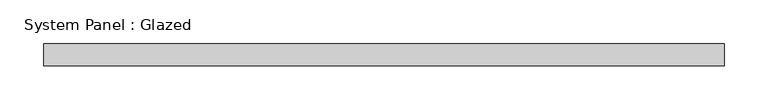
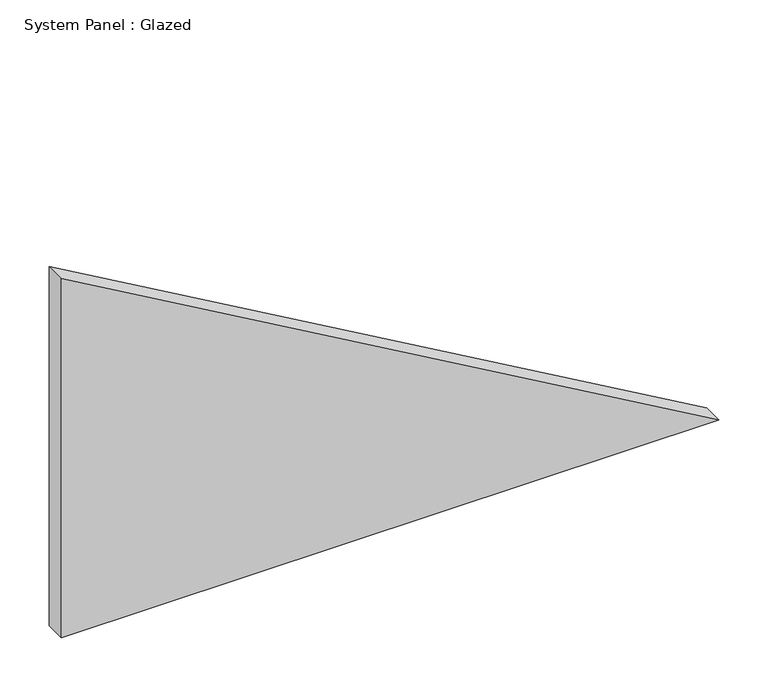
"""IFC4 building model written with IfcOpenShell, lengths in millimetres: plate geometry, System Panel : Glazed."""

from ifc_helpers import new_model, si_unit, frame, origin, place, context, project, spatial, polyline, outline, extrude, source, transform, mapped, element, save


def system_panel_glazed_7669df95(model_context):
    return source(origin(), model_context, "Body", "SweptSolid", [
        extrude(outline(polyline([(0.0, -387.4252157), (0.0, 387.4252157), (447.3601051, -387.4252157), (0.0, -387.4252157)])), frame((0.0, 24.5, 0.0), z_axis=(0.0, 1.0, 0.0), x_axis=(0.0, 0.0, 1.0)), (0.0, 0.0, 1.0), 25.0),
    ])


if __name__ == "__main__":
    model = new_model("IFC4")
    model_context = context("Model", 3, world=origin())
    ifc_project = project(units=[si_unit("LENGTHUNIT", "METRE", prefix="MILLI")], contexts=[model_context])
    site = spatial("IfcSite", under=ifc_project)
    building = spatial("IfcBuilding", under=site)
    placement = place(None, origin())
    system_panel_glazed_shape = system_panel_glazed_7669df95(model_context)
    element("IfcPlate", 1, ObjectType="System Panel : Glazed", at=placement, inside=building, context=model_context, shape_type="MappedRepresentation", body=[
        mapped(system_panel_glazed_shape, transform((0.0, 0.0, 0.0), x_axis=(1.0, 0.0, 0.0), y_axis=(0.0, 1.0, 0.0), z_axis=(0.0, 0.0, 1.0))),
    ])
    save(model, "model.ifc")

# Revit data of these elements
# Type "System Panel : Glazed"
#   Construction Type Id = "GSP4R"
#   Analytic Construction = "1/8 in Pilkington single glazing"
#   Visual Light Transmittance = 0.9
#   Solar Heat Gain Coefficient = 0.86
#   Heat Transfer Coefficient (U) = 6.7069 W/(m²·K)
#   Define Thermal Properties by = 1
# Element 1 (IfcPlate, "System Panel : Glazed")
#   Materials on its faces: "Glass"
# Materials
#   "Glass": class "Glass", colour RGB 0 128 192, transparency 0.75, Description = "Soda Lime Glass", Cost = 0
